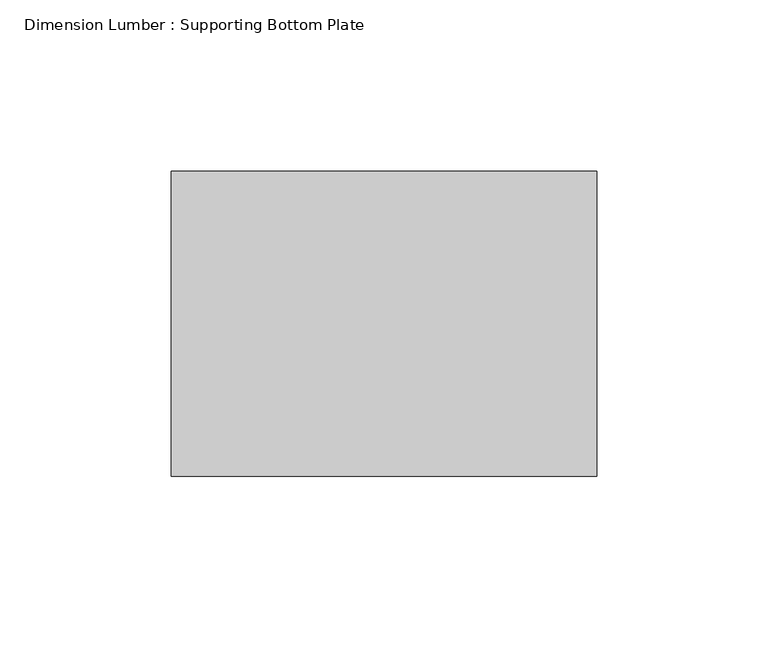
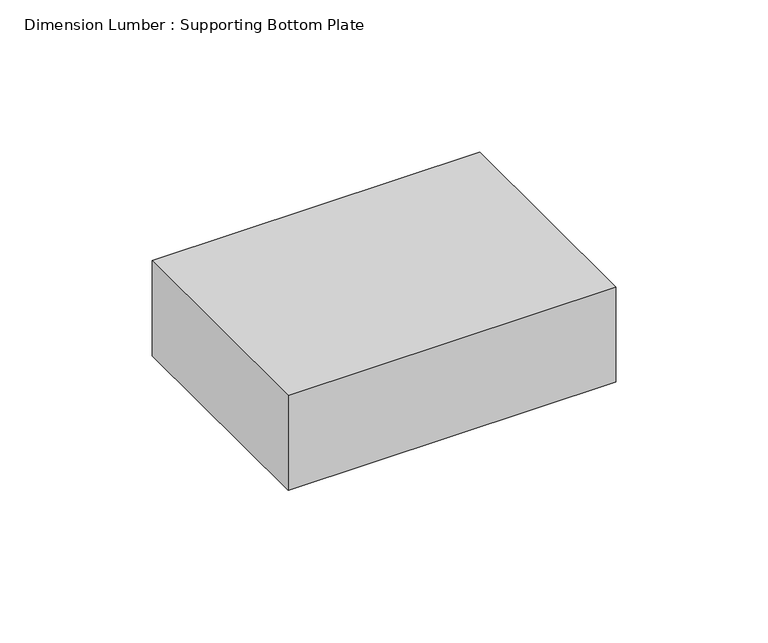
"""IFC4 building model written with IfcOpenShell, lengths in millimetres: beam geometry, Dimension Lumber : Supporting Bottom Plate."""

from ifc_helpers import new_model, si_unit, frame, origin, place, context, project, spatial, polyline, outline, extrude, source, transform, mapped, element, save


def dimension_lumber_supporting_bottom_plate_a3b44643(model_context):
    return source(origin(), model_context, "Body", "SweptSolid", [
        extrude(outline(polyline([(84.225, 44.45), (84.225, -44.45), (-39.775, -44.45), (-39.775, 44.45), (84.225, 44.45)])), frame((0.0, 0.0, -19.05), z_axis=(0.0, 0.0, 1.0), x_axis=(1.0, 0.0, 0.0)), (0.0, 0.0, 1.0), 38.1),
    ])


if __name__ == "__main__":
    model = new_model("IFC4")
    model_context = context("Model", 3, world=origin())
    ifc_project = project(units=[si_unit("LENGTHUNIT", "METRE", prefix="MILLI")], contexts=[model_context])
    site = spatial("IfcSite", under=ifc_project)
    building = spatial("IfcBuilding", under=site)
    placement = place(None, origin())
    dimension_lumber_supporting_bottom_plate_shape = dimension_lumber_supporting_bottom_plate_a3b44643(model_context)
    element("IfcBeam", 1, ObjectType="Dimension Lumber : Supporting Bottom Plate", at=placement, inside=building, context=model_context, shape_type="MappedRepresentation", body=[
        mapped(dimension_lumber_supporting_bottom_plate_shape, transform((0.0, 0.0, 0.0), x_axis=(1.0, 0.0, 0.0), y_axis=(0.0, 1.0, 0.0), z_axis=(0.0, 0.0, 1.0))),
    ])
    save(model, "model.ifc")

# Revit data of these elements
# Type "Dimension Lumber : Supporting Bottom Plate"
#   Assembly Code = "B10"
#   A = 0.0364583 SF
#   Length [instance default] = 5' - 0"
#   b = 0' - 3 1/2"
#   d = 0' - 1 1/2"
#   Structural Material [instance default] = Softwood, Lumber
# Element 1 (IfcBeam, "Dimension Lumber : Supporting Bottom Plate")
#   Structural Material = Douglas Fir #2
#   Materials on its faces: "Douglas Fir #2"
# Materials
#   "Softwood, Lumber": class "Wood", colour RGB 223 192 134, transparency 0, Description = "Pinus Echinata", Cost = 0
#   "Douglas Fir #2": class "Wood", colour RGB 223 192 134, transparency 0, Description = "Pinus Echinata", Cost = 0
